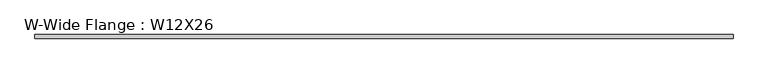
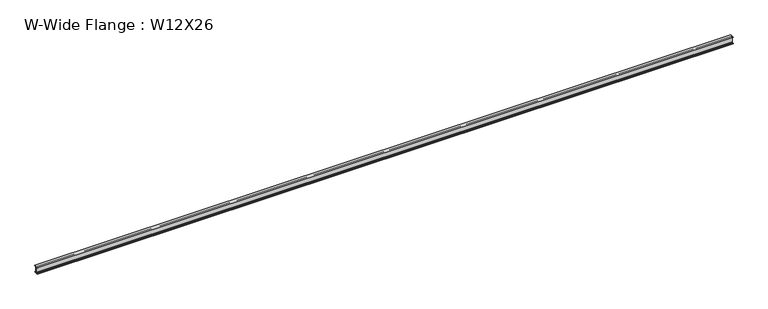
"""IFC4 building model written with IfcOpenShell, lengths in millimetres: beam geometry, W-Wide Flange : W12X26."""

from ifc_helpers import new_model, si_unit, point, frame, frame_2d, origin, place, context, project, spatial, polyline, circle_curve, trimmed, segment, composite_curve, outline, extrude, source, transform, mapped, element, save


def w_wide_flange_w12x26_862ffa42(model_context):
    return source(origin(), model_context, "Body", "SweptSolid", [
        extrude(outline(composite_curve([segment(polyline([(82.4011719, -145.5539063), (82.4011719, -155.178125), (-82.4011719, -155.178125), (-82.4011719, -145.5539063), (-20.2902344, -145.5539063)]), True, "CONTINUOUS"), segment(trimmed(circle_curve(frame_2d((-20.2902344, -128.190625)), 17.3632812), [point((-20.2902344, -145.5539063))], [point((-2.9269531, -128.190625))], True, "CARTESIAN"), True, "CONTINUOUS"), segment(polyline([(-2.9269531, -128.190625), (-2.9269531, 128.190625)]), True, "CONTINUOUS"), segment(trimmed(circle_curve(frame_2d((-20.2902344, 128.190625)), 17.3632812), [point((-2.9269531, 128.190625))], [point((-20.2902344, 145.5539062))], True, "CARTESIAN"), True, "CONTINUOUS"), segment(polyline([(-20.2902344, 145.5539062), (-82.4011719, 145.5539062), (-82.4011719, 155.178125), (82.4011719, 155.178125), (82.4011719, 145.5539062), (20.2902344, 145.5539062)]), True, "CONTINUOUS"), segment(trimmed(circle_curve(frame_2d((20.2902344, 128.190625)), 17.3632812), [point((20.2902344, 145.5539062))], [point((2.9269531, 128.190625))], True, "CARTESIAN"), True, "CONTINUOUS"), segment(polyline([(2.9269531, 128.190625), (2.9269531, -128.190625)]), True, "CONTINUOUS"), segment(trimmed(circle_curve(frame_2d((20.2902344, -128.190625)), 17.3632812), [point((2.9269531, -128.190625))], [point((20.2902344, -145.5539063))], True, "CARTESIAN"), True, "CONTINUOUS"), segment(polyline([(20.2902344, -145.5539063), (82.4011719, -145.5539063)]), True, "CONTINUOUS")], self_intersect=False)), frame((-29402.3785884, 0.0, 0.0), z_axis=(1.0, 0.0, 0.0), x_axis=(0.0, 1.0, 0.0)), (0.0, 0.0, 1.0), 31278.6693847),
    ])


if __name__ == "__main__":
    model = new_model("IFC4")
    model_context = context("Model", 3, world=origin())
    ifc_project = project(units=[si_unit("LENGTHUNIT", "METRE", prefix="MILLI")], contexts=[model_context])
    site = spatial("IfcSite", under=ifc_project)
    building = spatial("IfcBuilding", under=site)
    placement = place(None, origin())
    w_wide_flange_w12x26_shape = w_wide_flange_w12x26_862ffa42(model_context)
    element("IfcBeam", 1, ObjectType="W-Wide Flange : W12X26", at=placement, inside=building, context=model_context, shape_type="MappedRepresentation", body=[
        mapped(w_wide_flange_w12x26_shape, transform((0.0, 0.0, 0.0), x_axis=(1.0, 0.0, 0.0), y_axis=(0.0, 1.0, 0.0), z_axis=(0.0, 0.0, 1.0))),
    ])
    save(model, "model.ifc")

# Revit data of these elements
# Type "W-Wide Flange : W12X26"
#   Assembly Code = "B10"
#   W = 26
#   Length [instance default] = 5' - 0"
#   bf = 0' - 6 125/256"
#   d = 1' - 0 7/32"
#   k = 0' - 1 1/16"
#   k2 = 0' - 0 175/256"
#   tf = 0' - 0 97/256"
#   tw = 0' - 0 59/256"
#   A = 0.053125 SF
#   Structural Material [instance default] = none
